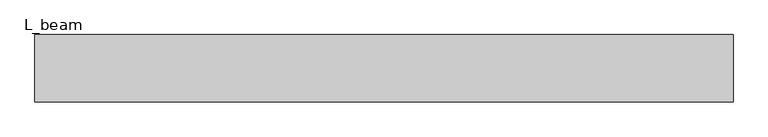
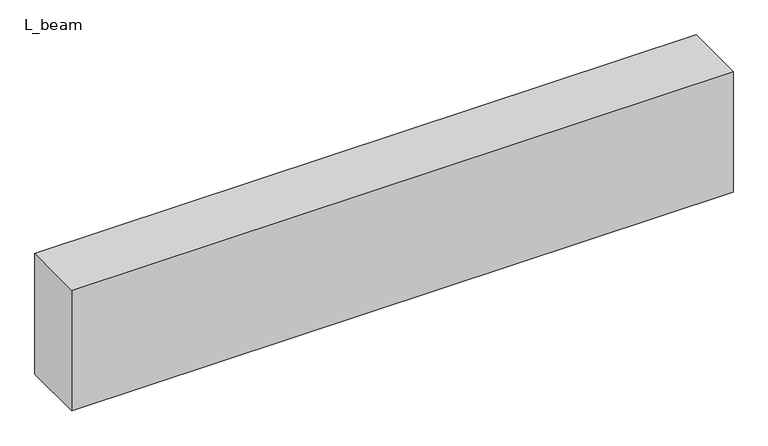
"""IFC4 building model written with IfcOpenShell, lengths in millimetres: beam geometry, 混凝土 - 矩形梁 : L_beam."""

from ifc_helpers import new_model, si_unit, frame, origin, place, context, project, spatial, polyline, outline, extrude, source, transform, mapped, element, save


def l_beam_a690bdf5(model_context):
    return source(origin(), model_context, "Body", "SweptSolid", [
        extrude(outline(polyline([(1555.0, 150.0), (1555.0, -150.0), (-1555.0, -150.0), (-1555.0, 150.0), (1555.0, 150.0)])), frame((0.0, 0.0, -300.0), z_axis=(0.0, 0.0, 1.0), x_axis=(1.0, 0.0, 0.0)), (0.0, 0.0, 1.0), 600.0),
    ])


if __name__ == "__main__":
    model = new_model("IFC4")
    model_context = context("Model", 3, world=origin())
    ifc_project = project(units=[si_unit("LENGTHUNIT", "METRE", prefix="MILLI")], contexts=[model_context])
    site = spatial("IfcSite", under=ifc_project)
    building = spatial("IfcBuilding", under=site)
    placement = place(None, origin())
    l_beam_shape = l_beam_a690bdf5(model_context)
    element("IfcBeam", 1, ObjectType="混凝土 - 矩形梁 : L_beam", at=placement, inside=building, context=model_context, shape_type="MappedRepresentation", body=[
        mapped(l_beam_shape, transform((0.0, 0.0, 0.0), x_axis=(1.0, 0.0, 0.0), y_axis=(0.0, 1.0, 0.0), z_axis=(0.0, 0.0, 1.0))),
    ])
    save(model, "model.ifc")

# Revit data of these elements
# Type "混凝土 - 矩形梁 : L_beam"
#   Length [instance default] = 1524 mm
#   b = 300 mm
#   h = 600 mm
#   Structural Material [instance default] = none
#   Assembly Code = ""
